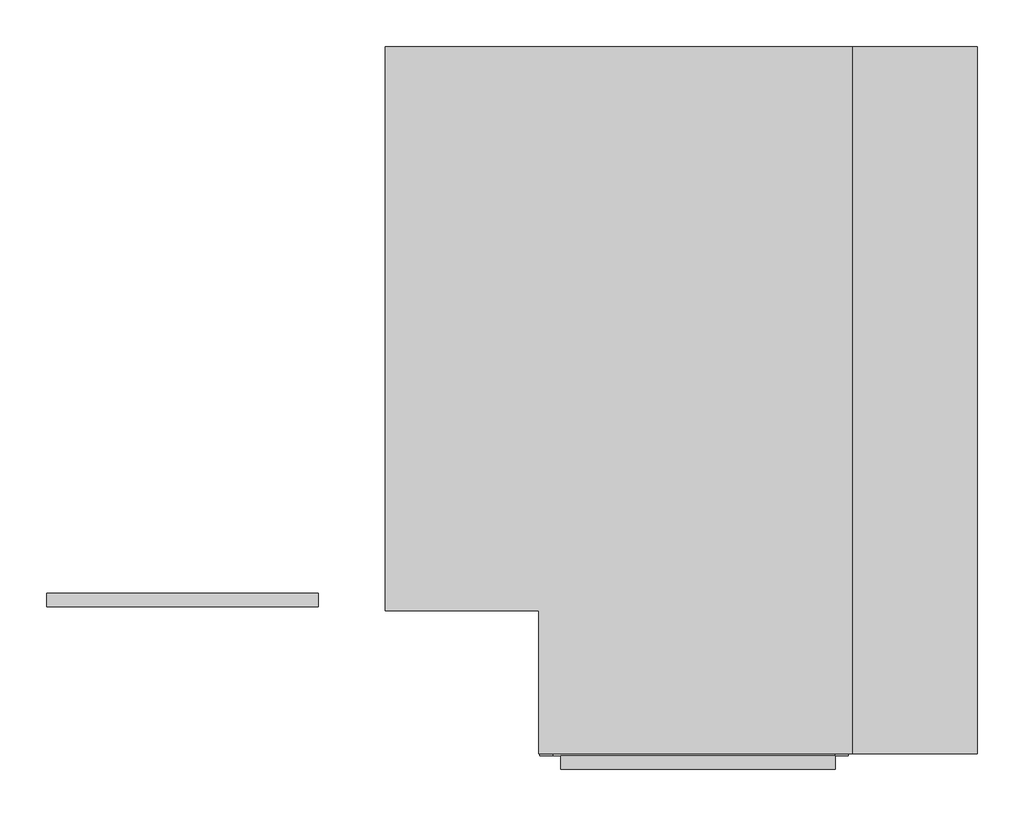
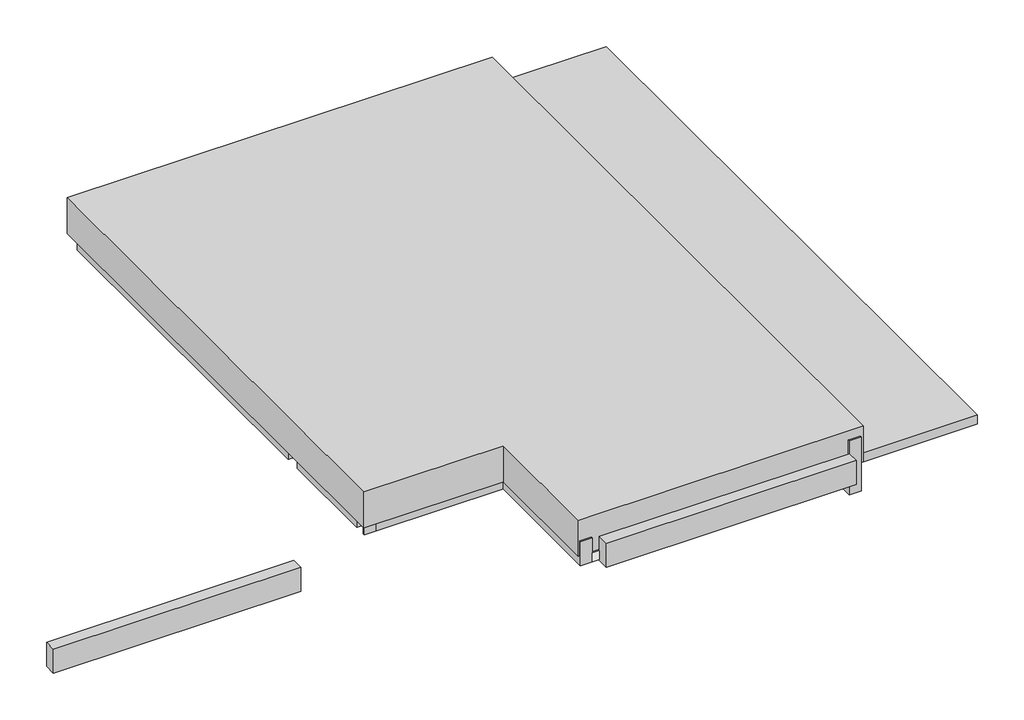
# One storey: 7 beams, 2 proxies, 2 slabs.
"""IFC4 building model written with IfcOpenShell, lengths in millimetres."""

from ifc_helpers import new_model, si_unit, frame, origin, place, context, project, spatial, polyline, circle_curve, ellipse_curve, outline, extrude, faceted_brep, element, save
from ifc_brep_helpers import plane_surface, cylinder_surface, revolved_surface, advanced_brep

model = new_model("IFC4")

# Units and contexts
model_context = context("Model", 3, world=origin())
ifc_project = project(units=[si_unit("LENGTHUNIT", "METRE", prefix="MILLI")], contexts=[model_context])

# Site, building, storey
site = spatial("IfcSite", under=ifc_project)
building = spatial("IfcBuilding", under=site)
storey = spatial("IfcBuildingStorey", under=building, Name="COBERTURA SALA DE ESTAR", Elevation=4400.0)

# Beams
placement = place(None, origin())
element("IfcBeam", 1, ObjectType="TQS - Viga retangular : 19.0 x 40.0", at=placement, inside=storey, context=model_context, shape_type="SweptSolid", body=[
    extrude(outline(polyline([(-7621.281307, -2044.5699847), (-7621.281307, -2234.5699847), (-11521.281307, -2234.5699847), (-11521.281307, -2044.5699847), (-7621.281307, -2044.5699847)])), frame((0.0, 0.0, 3640.0), z_axis=(0.0, 0.0, 1.0), x_axis=(1.0, 0.0, 0.0)), (0.0, 0.0, 1.0), 400.0),
])
element("IfcBeam", 2, ObjectType="TQS - Viga retangular : 19.0 x 40.0", at=placement, inside=storey, context=model_context, shape_type="SweptSolid", body=[
    extrude(outline(polyline([(-202.281307, -4375.5699847), (-202.281307, -4565.5699847), (-4142.481307, -4565.5699847), (-4142.481307, -4375.5699847), (-202.281307, -4375.5699847)])), frame((0.0, 0.0, 4240.0), z_axis=(0.0, 0.0, 1.0), x_axis=(1.0, 0.0, 0.0)), (0.0, 0.0, 1.0), 400.0),
])
element("IfcBeam", 3, ObjectType="TQS - Viga retangular : 19.0 x 40.0", at=placement, inside=storey, context=model_context, shape_type="Brep", body=[
    faceted_brep([(-4442.481307, -2259.5699847, 4650.0), (-4252.481307, -2259.5699847, 4650.0), (-4252.481307, -2259.5699847, 4400.0), (-4252.481307, -2259.5699847, 4250.0), (-4442.481307, -2259.5699847, 4250.0), (-4442.481307, -4375.5699847, 4650.0), (-4252.481307, -4375.5699847, 4650.0), (-4252.481307, -4375.5699847, 4400.0), (-4252.481307, -4375.5699847, 4250.0), (-4442.481307, -4375.5699847, 4250.0)], [[[0, 1, 2, 3, 4]], [[1, 0, 5, 6]], [[3, 2, 1, 6, 7, 8]], [[4, 3, 8, 9]], [[0, 4, 9, 5]], [[5, 9, 8, 7, 6]]]),
])
element("IfcBeam", 4, ObjectType="TQS - Viga retangular : 19.0 x 60.0", at=placement, inside=storey, context=model_context, shape_type="AdvancedBrep", body=[
    advanced_brep(
    [(-412.281307, 5774.4300153, 4850.0), (-6230.281307, 5774.4300153, 4850.0), (-6230.281307, 5620.2264681, 4850.0), (-6139.9212645, 5625.5330018, 4850.0), (-6117.841019, 5621.0415768, 4850.0), (-6230.281307, 5613.9936641, 4850.0), (-6230.281307, 5584.4300153, 4850.0), (-412.281307, 5584.4300153, 4850.0), (-412.281307, 5610.6528241, 4850.0), (-563.721595, 5621.0415768, 4850.0), (-541.6413494, 5625.5330018, 4850.0), (-412.281307, 5617.2895263, 4850.0), (-6230.281307, 5584.4300153, 4250.0), (-412.281307, 5584.4300153, 4250.0), (-6230.281307, 5774.4300153, 4250.0), (-412.281307, 5774.4300153, 4250.0), (-6230.281307, 5621.0415768, 4838.7559712), (-6230.281307, 5625.5330018, 4840.9639958), (-412.281307, 5625.5330018, 4837.0639958), (-412.281307, 5621.0415768, 4834.8559712)],
    [
        (0, 1),
        (1, 2),
        (2, 3, ellipse_curve(frame((-5844.9559183, 5565.5330018, 4850.0), z_axis=(0.0, 0.0, -1.0), x_axis=(-0.9999999999999999, 0.0, 0.0)), 671.270851, 66.7939461)),
        (3, 4),
        (4, 5, ellipse_curve(frame((-5844.9559183, 5565.5330018, 4850.0), z_axis=(0.0, 0.0, 1.0), x_axis=(-0.9999999999999999, 0.0, 0.0)), 621.0214729, 61.7939461)),
        (5, 6),
        (6, 7),
        (7, 8),
        (8, 9, ellipse_curve(frame((-836.6066956, 5565.5330018, 4850.0), z_axis=(0.0, 0.0, 1.0), x_axis=(-0.9999999999999999, 0.0, 0.0)), 621.0214729, 61.7939461)),
        (9, 10),
        (10, 11, ellipse_curve(frame((-836.6066956, 5565.5330018, 4850.0), z_axis=(0.0, 0.0, -1.0), x_axis=(-0.9999999999999999, 0.0, 0.0)), 671.270851, 66.7939461)),
        (11, 0),
        (6, 12),
        (12, 13),
        (13, 7),
        (12, 14),
        (14, 15),
        (15, 13),
        (0, 15),
        (14, 1),
        (5, 16, ellipse_curve(frame((-6230.281307, 5565.5330018, 4811.4674611), z_axis=(-1.0, 0.0, 0.0), x_axis=(0.0, 0.0, -1.0)), 62.1021473, 61.7939461)),
        (16, 17),
        (17, 2, ellipse_curve(frame((-6230.281307, 5565.5330018, 4811.4674611), z_axis=(1.0, 0.0, 0.0), x_axis=(0.0, 0.0, -1.0)), 67.1270851, 66.7939461)),
        (11, 18, ellipse_curve(frame((-412.281307, 5565.5330018, 4807.5674611), z_axis=(-1.0, 0.0, 0.0), x_axis=(0.0, 0.0, 1.0)), 67.1270851, 66.7939461)),
        (18, 19),
        (19, 8, ellipse_curve(frame((-412.281307, 5565.5330018, 4807.5674611), z_axis=(1.0, 0.0, 0.0), x_axis=(0.0, 0.0, 1.0)), 62.1021473, 61.7939461)),
        (4, 16),
        (3, 17),
        (19, 9),
        (18, 10),
    ],
    [
        plane_surface(frame((-424.9813076, 5774.4300153, 4850.0), z_axis=(0.0, 0.0, 1.0), x_axis=(-1.0, 0.0, 0.0))),
        plane_surface(frame((-424.9813076, 5584.4300153, 4850.0), z_axis=(0.0, -1.0, 0.0), x_axis=(-1.0, 0.0, 0.0))),
        plane_surface(frame((-424.9813076, 5584.4300153, 4250.0), z_axis=(0.0, 0.0, -1.0), x_axis=(-1.0, 0.0, 0.0))),
        plane_surface(frame((-424.9813076, 5774.4300153, 4250.0), z_axis=(0.0, 1.0, 0.0), x_axis=(-1.0, 0.0, 0.0))),
        plane_surface(frame((-6230.281307, 5679.4300153, 4850.0), z_axis=(-1.0, 0.0, 0.0), x_axis=(0.0, -1.0, 0.0))),
        plane_surface(frame((-412.281307, 5679.4300153, 4850.0), z_axis=(1.0, 0.0, 0.0), x_axis=(0.0, 1.0, 0.0))),
        cylinder_surface(frame((-3344.074248, 5565.5330018, 5100.088167), z_axis=(-0.9950371902099892, 0.0, -0.09950371902099951), x_axis=(-0.0893826983688466, 0.4394133093826145, 0.8938269836885228)), 61.7939461),
        plane_surface(frame((-3346.8853889, 5623.2872893, 5128.1995753), z_axis=(-0.08938269836887112, -0.4394133093823482, 0.8938269836886512), x_axis=(-0.043723258470857625, 0.8982850012872601, 0.4372325847086854))),
        revolved_surface(polyline([(-6515.550746384648, 5536.182852897475, 4843.239770846461), (-5186.301536483657, 5536.182852897475, 4976.164691836561)]), (-3344.074248, 5565.5330018, 5100.088167), (-0.9950371902099892, 0.0, -0.09950371902099951)),
        cylinder_surface(frame((-379.7327874, 5565.5330018, 4804.3126092), z_axis=(-0.9950371902099892, 0.0, 0.09950371902099964), x_axis=(0.08938269836885342, 0.43941330938261464, 0.893826983688522)), 61.7939461),
        plane_surface(frame((-376.9216465, 5623.2872893, 4832.4240174), z_axis=(0.08938269836886582, -0.43941330938234807, 0.8938269836886518), x_axis=(0.04372325847086866, 0.8982850012872601, 0.4372325847086842))),
        revolved_surface(polyline([(-1495.2610774113932, 5536.182852897475, 4976.164691886069), (-166.01186751040316, 5536.182852897475, 4843.239770895969)]), (-379.7327874, 5565.5330018, 4804.3126092), (-0.9950371902099892, 0.0, 0.09950371902099964)),
    ],
    [
        (0, [[1, 2, 3, 4, 5, 6, 7, 8, 9, 10, 11, 12]]),
        (1, [[-7, 13, 14, 15]]),
        (2, [[-14, 16, 17, 18]]),
        (3, [[-1, 19, -17, 20]]),
        (4, [[-20, -16, -13, -6, 21, 22, 23, -2]]),
        (5, [[-15, -18, -19, -12, 24, 25, 26, -8]]),
        (6, [[27, -21, -5]]),
        (7, [[-27, -4, 28, -22]]),
        (8, [[-28, -3, -23]]),
        (9, [[29, -9, -26]]),
        (10, [[-29, -25, 30, -10]]),
        (11, [[-30, -24, -11]]),
    ],
),
])
element("IfcBeam", 5, ObjectType="TQS - Viga retangular : 19.0 x 60.0", at=placement, inside=storey, context=model_context, shape_type="Brep", body=[
    faceted_brep([(-6630.281307, -174.5699847, 4850.0), (-6440.281307, -174.5699847, 4850.0), (-6440.281307, 5584.4300153, 4850.0), (-6630.281307, 5584.4300153, 4850.0), (-6440.281307, -174.5699847, 4250.0), (-6440.281307, 5584.4300153, 4250.0), (-6440.281307, 5584.4300153, 4400.0), (-6630.281307, -174.5699847, 4250.0), (-6630.281307, 5584.4300153, 4250.0)], [[[0, 1, 2, 3]], [[1, 4, 5, 6, 2]], [[4, 7, 8, 5]], [[7, 0, 3, 8]], [[1, 0, 7, 4]], [[3, 2, 6, 5, 8]]]),
    faceted_brep([(-6630.281307, -424.5699847, 4850.0), (-6440.281307, -424.5699847, 4850.0), (-6440.281307, -424.5699847, 4250.0), (-6630.281307, -424.5699847, 4250.0), (-6630.281307, -2044.5699847, 4850.0), (-6440.281307, -2044.5699847, 4850.0), (-6440.281307, -2044.5699847, 4250.0), (-6630.281307, -2044.5699847, 4250.0)], [[[0, 1, 2, 3]], [[1, 0, 4, 5]], [[2, 1, 5, 6]], [[3, 2, 6, 7]], [[0, 3, 7, 4]], [[5, 4, 7, 6]]]),
    faceted_brep([(-6440.281307, -2259.5699847, 4850.0), (-6630.281307, -2259.5699847, 4850.0), (-6630.281307, -2259.5699847, 4250.0), (-6440.281307, -2259.5699847, 4250.0), (-6630.281307, -2234.5699847, 4850.0), (-6440.281307, -2234.5699847, 4850.0), (-6440.281307, -2234.5699847, 4250.0), (-6630.281307, -2234.5699847, 4250.0)], [[[0, 1, 2, 3]], [[4, 5, 6, 7]], [[1, 0, 5, 4]], [[0, 3, 6, 5]], [[3, 2, 7, 6]], [[2, 1, 4, 7]]]),
])
element("IfcBeam", 6, ObjectType="TQS - Viga retangular : 19.0 x 60.0", at=placement, inside=storey, context=model_context, shape_type="AdvancedBrep", body=[
    advanced_brep(
    [(-202.6220088, -2259.5699847, 4850.0), (-202.6137562, -2069.5699847, 4850.0), (-6440.281307, -2069.5699847, 4850.0), (-6440.281307, -2234.5699847, 4850.0), (-6440.281307, -2259.5699847, 4850.0), (-375.1640483, -2209.9569973, 4850.0), (-375.1640483, -2217.1114577, 4850.0), (-563.721595, -2202.9584232, 4850.0), (-541.6413494, -2198.4669982, 4850.0), (-202.6220088, -2259.5699847, 4250.0), (-202.6220088, -2259.5699847, 4400.0), (-6440.281307, -2259.5699847, 4250.0), (-4442.481307, -2259.5699847, 4250.0), (-4252.481307, -2259.5699847, 4250.0), (-202.6137562, -2069.5699847, 4250.0), (-6440.281307, -2234.5699847, 4250.0), (-6440.281307, -2069.5699847, 4250.0), (-202.6137562, -2069.5699847, 4400.0), (-6440.281307, -2069.5699847, 4400.0), (-376.8123384, -2198.4669982, 4833.5170989), (-377.0309547, -2202.9584232, 4831.330936)],
    [
        (0, 1),
        (1, 2),
        (2, 3),
        (3, 4),
        (4, 0),
        (5, 6),
        (6, 7, ellipse_curve(frame((-836.6066956, -2258.4669982, 4850.0), z_axis=(0.0, 0.0, 1.0), x_axis=(-0.9999999999999999, 0.0, 0.0)), 621.0214729, 61.7939461)),
        (7, 8),
        (8, 5, ellipse_curve(frame((-836.6066956, -2258.4669982, 4850.0), z_axis=(0.0, 0.0, -1.0), x_axis=(-0.9999999999999999, 0.0, 0.0)), 671.270851, 66.7939461)),
        (9, 10),
        (10, 0),
        (4, 11),
        (11, 12),
        (12, 13),
        (13, 9),
        (14, 9),
        (11, 15),
        (15, 16),
        (16, 14),
        (1, 17),
        (17, 14),
        (16, 18),
        (18, 2),
        (19, 20),
        (20, 6, circle_curve(frame((-379.7327874, -2258.4669982, 4804.3126092), z_axis=(0.9950371902099892, 0.0, -0.09950371902099961), x_axis=(0.08938269836885339, 0.4394133093826145, 0.893826983688522)), 61.7939461)),
        (5, 19, circle_curve(frame((-379.7327874, -2258.4669982, 4804.3126092), z_axis=(-0.9950371902099892, 0.0, 0.09950371902099961), x_axis=(0.08938269836885117, -0.4394133093826303, 0.8938269836885144)), 66.7939461)),
        (20, 7),
        (19, 8),
    ],
    [
        plane_surface(frame((-215.3220088, -2069.5699847, 4850.0), z_axis=(0.0, 0.0, 1.0), x_axis=(-1.0, 0.0, 0.0))),
        plane_surface(frame((-215.3220088, -2259.5699847, 4850.0), z_axis=(0.0, -1.0, 0.0), x_axis=(-1.0, 0.0, 0.0))),
        plane_surface(frame((-215.3220088, -2259.5699847, 4250.0), z_axis=(0.0, 0.0, -1.0), x_axis=(-1.0, 0.0, 0.0))),
        plane_surface(frame((-215.3220088, -2069.5699847, 4250.0), z_axis=(0.0, 1.0, 0.0), x_axis=(-1.0, 0.0, 0.0))),
        plane_surface(frame((-6440.281307, -2234.5699847, 4850.0), z_axis=(-1.0, 0.0, 0.0), x_axis=(0.0, 0.0, -1.0))),
        plane_surface(frame((-202.2818588, 5571.7300153, 3950.0), z_axis=(0.9999999990567141, -4.343468567533895e-05, 0.0), x_axis=(-4.343468567533895e-05, -0.9999999990567141, 0.0))),
        plane_surface(frame((-373.8918894, -2311.673052, 4862.7215886), z_axis=(-0.9950371902099892, 0.0, 0.09950371902099943), x_axis=(-0.09950371902099943, 0.0, -0.9950371902099892))),
        cylinder_surface(frame((-379.7327874, -2258.4669982, 4804.3126092), z_axis=(-0.9950371902099892, 0.0, 0.09950371902099961), x_axis=(0.08938269836885339, 0.4394133093826145, 0.893826983688522)), 61.7939461),
        plane_surface(frame((-376.9216465, -2200.7127107, 4832.4240174), z_axis=(0.0893826983688658, -0.4394133093823482, 0.8938269836886518), x_axis=(0.04372325847086866, 0.8982850012872601, 0.4372325847086843))),
        revolved_surface(polyline([(-1495.2610774113932, -2287.817147102526, 4976.164691886069), (-166.01186751040316, -2287.817147102526, 4843.239770895969)]), (-379.7327874, -2258.4669982, 4804.3126092), (-0.9950371902099892, 0.0, 0.09950371902099961)),
    ],
    [
        (0, [[1, 2, 3, 4, 5], [6, 7, 8, 9]]),
        (1, [[10, 11, -5, 12, 13, 14, 15]]),
        (2, [[16, -15, -14, -13, 17, 18, 19]]),
        (3, [[20, 21, -19, 22, 23, -2]]),
        (4, [[-23, -22, -18, -17, -12, -4, -3]]),
        (5, [[-1, -11, -10, -16, -21, -20]]),
        (6, [[24, 25, -6, 26]]),
        (7, [[-25, 27, -7]]),
        (8, [[-24, 28, -8, -27]]),
        (9, [[-26, -9, -28]]),
    ],
),
])
element("IfcBeam", 7, ObjectType="TQS - Viga retangular : 19.0 x 90.0", at=placement, inside=storey, context=model_context, shape_type="Brep", body=[
    faceted_brep([(-12.281307, 5584.4300153, 4850.0), (-202.2813068, 5584.4382679, 4850.0), (-202.6137562, -2069.5699847, 4850.0), (-202.6220088, -2259.5699847, 4850.0), (-202.7139163, -4375.561732, 4850.0), (-12.7139164, -4375.5699846, 4850.0), (-12.281307, 5584.4300153, 3950.0), (-12.7139164, -4375.5699846, 3950.0), (-202.2813068, 5584.4382679, 3950.0), (-202.7139163, -4375.561732, 3950.0)], [[[0, 1, 2, 3, 4, 5]], [[6, 0, 5, 7]], [[8, 6, 7, 9]], [[1, 8, 9, 4, 3, 2]], [[1, 0, 6, 8]], [[4, 9, 7, 5]]]),
])

# Proxies
element("IfcBuildingElementProxy", 8, Name="PERGOLADO SALAS1 : PERGOLADO SALAS", ObjectType="PERGOLADO SALAS1 : PERGOLADO SALAS", at=placement, inside=storey, context=model_context, shape_type="SweptSolid", body=[
    extrude(outline(polyline([(1839.718693, 5804.4300153), (1839.718693, -4345.5699847), (39.718693, -4345.5699847), (39.718693, 5804.4300153), (1839.718693, 5804.4300153)])), frame((0.0, 0.0, 4400.0), z_axis=(0.0, 0.0, 1.0), x_axis=(1.0, 0.0, 0.0)), (0.0, 0.0, 1.0), 150.0),
])
element("IfcBuildingElementProxy", 9, Name="COBERTURA SALA DE ESTAR : COBERTURA SALA DE ESTAR", ObjectType="COBERTURA SALA DE ESTAR : COBERTURA SALA DE ESTAR", at=placement, inside=storey, context=model_context, shape_type="SweptSolid", body=[
    extrude(outline(polyline([(39.718693, 5804.4300153), (39.718693, -4345.5699847), (-4457.4976512, -4345.5699847), (-4457.4976512, -2295.5699847), (-6660.281307, -2295.5699847), (-6660.281307, 5804.4300153), (39.718693, 5804.4300153)])), frame((0.0, 0.0, 4400.0), z_axis=(0.0, 0.0, 1.0), x_axis=(1.0, 0.0, 0.0)), (0.0, 0.0, 1.0), 600.0),
])

# Slabs
element("IfcSlab", 10, ObjectType="TQS h=15", at=placement, inside=storey, context=model_context, shape_type="Brep", body=[
    faceted_brep([(-6440.281307, -2069.5699847, 4250.0), (-6440.281307, -2044.5699847, 4250.0), (-6440.281307, -424.5699847, 4250.0), (-6440.281307, -174.5699847, 4250.0), (-6440.281307, 5584.4300153, 4250.0), (-6230.281307, 5584.4300153, 4250.0), (-412.281307, 5584.4300153, 4250.0), (-202.2813071, 5584.4300153, 4250.0), (-202.6137562, -2069.5699847, 4250.0), (-6440.281307, -2069.5699847, 4400.0), (-202.6137562, -2069.5699847, 4400.0), (-202.2813071, 5584.4300153, 4400.0), (-6440.281307, 5584.4300153, 4400.0)], [[[0, 1, 2, 3, 4, 5, 6, 7, 8]], [[9, 10, 11, 12]], [[4, 3, 2, 1, 0, 9, 12]], [[7, 6, 5, 4, 12, 11]], [[8, 7, 11, 10]], [[0, 8, 10, 9]]]),
])
element("IfcSlab", 11, ObjectType="TQS h=15", at=placement, inside=storey, context=model_context, shape_type="SweptSolid", body=[
    extrude(outline(polyline([(-202.6220088, -2259.5699847), (-202.7139166, -4375.5699847), (-4252.481307, -4375.5699847), (-4252.481307, -2259.5699847), (-202.6220088, -2259.5699847)])), frame((0.0, 0.0, 4250.0), z_axis=(0.0, 0.0, 1.0), x_axis=(1.0, 0.0, 0.0)), (0.0, 0.0, 1.0), 150.0),
])

save(model, "model.ifc")

# Revit data of these elements
# Type "TQS - Viga retangular : 19.0 x 40.0"
#   Length [instance default] = 1.524 m
#   b = 0.19 m
#   h = 0.40 m
#   Structural Material [instance default] = none
#   Assembly Code = ""
# Type "TQS - Viga retangular : 19.0 x 60.0"
#   Length [instance default] = 1.524 m
#   b = 0.19 m
#   h = 0.60 m
#   Structural Material [instance default] = none
#   Assembly Code = ""
# Type "TQS - Viga retangular : 19.0 x 90.0"
#   Length [instance default] = 1.524 m
#   b = 0.19 m
#   h = 0.90 m
#   Structural Material [instance default] = none
#   Assembly Code = ""
# Type "TQS h=15"
#   Function = 0
#   Layers, outside or top first: 0.15 m ".MATERIAL GENÉRICO LAJE E PISO" (function 1)
# Element 1 (IfcBeam, "TQS - Viga retangular : 19.0 x 40.0")
#   Uso = "ESTRUTURA"
#   Titulo = "V302"
#   Chave = "-194"
#   Tipo Elemento = "Viga"
#   SHA1 = "623FD7AF7D5DA8F9D9CA08F45AA7E3989112ED0B"
#   Revisão = ""
#   Tipo de carga = ""
#   Divisor de flexao = ""
#   Secao = ""
#   Configuracao = ""
#   Angulo (graus) = ""
#   Detalhamento = ""
#   Casos de vento manual = ""
#   Tipo = ""
#   Alcas = ""
#   Furos = ""
#   Pino = ""
#   Distribuicao = ""
#   Solidarizado = ""
#   Solidarizar na montagem = ""
#   Unir com o próximo = ""
#   Grupo pre moldado = ""
#   Verificado = ""
#   Concreto C = ""
#   Taxa de armadura (kgf/m³) = 0
#   Carga (tf/m²) = 0
#   Carga (tf/m) = 0
#   Carga (tf) = 0
#   Altura = 0.40 m
#   Rebaixo = 0.36 m
#   Largura = 0.19 m
#   Distancia a face = 0.00 m
#   Distancia ao eixo = 0.00 m
#   Altura gerber esquerda = 0.00 m
#   Largura gerber esquerda = 0.00 m
#   Altura gerber direita = 0.00 m
#   Largura gerber direita = 0.00 m
#   Resultado de Ensaios fck (MPa) = 0
#   Unique TQS ID = -194
#   Principal = yes
#   Structural Material = none
#   Phase Created = CC_AP/ESTR
# Element 2 (IfcBeam, "TQS - Viga retangular : 19.0 x 40.0")
#   Uso = "ESTRUTURA"
#   Titulo = "V304"
#   Chave = "-347"
#   Tipo Elemento = "Viga"
#   SHA1 = "DE726C8B00042777CE20FAEC480409A8753BC175"
#   Revisão = ""
#   Tipo de carga = ""
#   Divisor de flexao = ""
#   Secao = ""
#   Configuracao = ""
#   Angulo (graus) = ""
#   Detalhamento = ""
#   Casos de vento manual = ""
#   Tipo = ""
#   Alcas = ""
#   Furos = ""
#   Pino = ""
#   Distribuicao = ""
#   Solidarizado = ""
#   Solidarizar na montagem = ""
#   Unir com o próximo = ""
#   Grupo pre moldado = ""
#   Verificado = ""
#   Concreto C = ""
#   Taxa de armadura (kgf/m³) = 0
#   Carga (tf/m²) = 0
#   Carga (tf/m) = 0
#   Carga (tf) = 0
#   Altura = 0.40 m
#   Rebaixo = -0.24 m
#   Largura = 0.19 m
#   Distancia a face = 0.00 m
#   Distancia ao eixo = 0.00 m
#   Altura gerber esquerda = 0.00 m
#   Largura gerber esquerda = 0.00 m
#   Altura gerber direita = 0.00 m
#   Largura gerber direita = 0.00 m
#   Resultado de Ensaios fck (MPa) = 0
#   Unique TQS ID = -347
#   Principal = yes
#   Structural Material = none
#   Phase Created = CC_AP/ESTR
# Element 3 (IfcBeam, "TQS - Viga retangular : 19.0 x 40.0")
#   Uso = "ESTRUTURA"
#   Titulo = "V306"
#   Chave = "-348"
#   Tipo Elemento = "Viga"
#   SHA1 = "0486A55721C7CA422F82DF13CBABE904850BDE6D"
#   Revisão = ""
#   Tipo de carga = ""
#   Divisor de flexao = ""
#   Secao = ""
#   Configuracao = ""
#   Angulo (graus) = ""
#   Detalhamento = ""
#   Casos de vento manual = ""
#   Tipo = ""
#   Alcas = ""
#   Furos = ""
#   Pino = ""
#   Distribuicao = ""
#   Solidarizado = ""
#   Solidarizar na montagem = ""
#   Unir com o próximo = ""
#   Grupo pre moldado = ""
#   Verificado = ""
#   Concreto C = ""
#   Taxa de armadura (kgf/m³) = 0
#   Carga (tf/m²) = 0
#   Carga (tf/m) = 0
#   Carga (tf) = 0
#   Altura = 0.40 m
#   Rebaixo = -0.25 m
#   Largura = 0.19 m
#   Distancia a face = 0.00 m
#   Distancia ao eixo = 0.00 m
#   Altura gerber esquerda = 0.00 m
#   Largura gerber esquerda = 0.00 m
#   Altura gerber direita = 0.00 m
#   Largura gerber direita = 0.00 m
#   Resultado de Ensaios fck (MPa) = 0
#   Unique TQS ID = -348
#   Principal = yes
#   Structural Material = none
#   Phase Created = CC_AP/ESTR
# Element 4 (IfcBeam, "TQS - Viga retangular : 19.0 x 60.0")
#   Uso = "ESTRUTURA"
#   Titulo = "V301"
#   Chave = "-296"
#   Tipo Elemento = "Viga"
#   SHA1 = "757894CEA72A4CB6221DF2E576041B09F085C368"
#   Revisão = ""
#   Tipo de carga = ""
#   Divisor de flexao = ""
#   Secao = ""
#   Configuracao = ""
#   Angulo (graus) = ""
#   Detalhamento = ""
#   Casos de vento manual = ""
#   Tipo = ""
#   Alcas = ""
#   Furos = ""
#   Pino = ""
#   Distribuicao = ""
#   Solidarizado = ""
#   Solidarizar na montagem = ""
#   Unir com o próximo = ""
#   Grupo pre moldado = ""
#   Verificado = ""
#   Concreto C = ""
#   Taxa de armadura (kgf/m³) = 0
#   Carga (tf/m²) = 0
#   Carga (tf/m) = 0
#   Carga (tf) = 0
#   Altura = 0.60 m
#   Rebaixo = -0.45 m
#   Largura = 0.19 m
#   Distancia a face = 0.00 m
#   Distancia ao eixo = 0.00 m
#   Altura gerber esquerda = 0.00 m
#   Largura gerber esquerda = 0.00 m
#   Altura gerber direita = 0.00 m
#   Largura gerber direita = 0.00 m
#   Resultado de Ensaios fck (MPa) = 0
#   Unique TQS ID = -296
#   Principal = yes
#   Structural Material = none
#   Phase Created = CC_AP/ESTR
# Element 5 (IfcBeam, "TQS - Viga retangular : 19.0 x 60.0")
#   Uso = "ESTRUTURA"
#   Titulo = "V305"
#   Chave = "-297"
#   Tipo Elemento = "Viga"
#   SHA1 = "BDE1024E341324ECB798242B9C26029271E807E6"
#   Revisão = ""
#   Tipo de carga = ""
#   Divisor de flexao = ""
#   Secao = ""
#   Configuracao = ""
#   Angulo (graus) = ""
#   Detalhamento = ""
#   Casos de vento manual = ""
#   Tipo = ""
#   Alcas = ""
#   Furos = ""
#   Pino = ""
#   Distribuicao = ""
#   Solidarizado = ""
#   Solidarizar na montagem = ""
#   Unir com o próximo = ""
#   Grupo pre moldado = ""
#   Verificado = ""
#   Concreto C = ""
#   Taxa de armadura (kgf/m³) = 0
#   Carga (tf/m²) = 0
#   Carga (tf/m) = 0
#   Carga (tf) = 0
#   Altura = 0.60 m
#   Rebaixo = -0.45 m
#   Largura = 0.19 m
#   Distancia a face = 0.00 m
#   Distancia ao eixo = 0.00 m
#   Altura gerber esquerda = 0.00 m
#   Largura gerber esquerda = 0.00 m
#   Altura gerber direita = 0.00 m
#   Largura gerber direita = 0.00 m
#   Resultado de Ensaios fck (MPa) = 0
#   Unique TQS ID = -297
#   Principal = yes
#   Structural Material = none
#   Phase Created = CC_AP/ESTR
# Element 6 (IfcBeam, "TQS - Viga retangular : 19.0 x 60.0")
#   Uso = "ESTRUTURA"
#   Titulo = "V303"
#   Chave = "-345"
#   Tipo Elemento = "Viga"
#   SHA1 = "033B8EC3397B601DC3ABF9BA590BF3ACBC45E410"
#   Revisão = ""
#   Tipo de carga = ""
#   Divisor de flexao = ""
#   Secao = ""
#   Configuracao = ""
#   Angulo (graus) = ""
#   Detalhamento = ""
#   Casos de vento manual = ""
#   Tipo = ""
#   Alcas = ""
#   Furos = ""
#   Pino = ""
#   Distribuicao = ""
#   Solidarizado = ""
#   Solidarizar na montagem = ""
#   Unir com o próximo = ""
#   Grupo pre moldado = ""
#   Verificado = ""
#   Concreto C = ""
#   Taxa de armadura (kgf/m³) = 0
#   Carga (tf/m²) = 0
#   Carga (tf/m) = 0
#   Carga (tf) = 0
#   Altura = 0.60 m
#   Rebaixo = -0.45 m
#   Largura = 0.19 m
#   Distancia a face = 0.00 m
#   Distancia ao eixo = 0.00 m
#   Altura gerber esquerda = 0.00 m
#   Largura gerber esquerda = 0.00 m
#   Altura gerber direita = 0.00 m
#   Largura gerber direita = 0.00 m
#   Resultado de Ensaios fck (MPa) = 0
#   Unique TQS ID = -345
#   Principal = yes
#   Structural Material = none
#   Phase Created = CC_AP/ESTR
# Element 7 (IfcBeam, "TQS - Viga retangular : 19.0 x 90.0")
#   Uso = "ESTRUTURA"
#   Titulo = "V307"
#   Chave = "-298"
#   Tipo Elemento = "Viga"
#   SHA1 = "4A4DC69E98A9D766DC72AD6B038202D9AEA1F49E"
#   Revisão = ""
#   Tipo de carga = ""
#   Divisor de flexao = ""
#   Secao = ""
#   Configuracao = ""
#   Angulo (graus) = ""
#   Detalhamento = ""
#   Casos de vento manual = ""
#   Tipo = ""
#   Alcas = ""
#   Furos = ""
#   Pino = ""
#   Distribuicao = ""
#   Solidarizado = ""
#   Solidarizar na montagem = ""
#   Unir com o próximo = ""
#   Grupo pre moldado = ""
#   Verificado = ""
#   Concreto C = ""
#   Taxa de armadura (kgf/m³) = 0
#   Carga (tf/m²) = 0
#   Carga (tf/m) = 0
#   Carga (tf) = 0
#   Altura = 0.90 m
#   Rebaixo = -0.45 m
#   Largura = 0.19 m
#   Distancia a face = 0.00 m
#   Distancia ao eixo = 0.00 m
#   Altura gerber esquerda = 0.00 m
#   Largura gerber esquerda = 0.00 m
#   Altura gerber direita = 0.00 m
#   Largura gerber direita = 0.00 m
#   Resultado de Ensaios fck (MPa) = 0
#   Unique TQS ID = -298
#   Principal = yes
#   Structural Material = none
#   Phase Created = CC_AP/ESTR
# Element 8 (IfcBuildingElementProxy, "PERGOLADO SALAS1 : PERGOLADO SALAS")
#   Phase Created = CC_COMPLETO
#   Materials on its faces: "Forma padrão"
# Element 9 (IfcBuildingElementProxy, "COBERTURA SALA DE ESTAR : COBERTURA SALA DE ESTAR")
#   Phase Created = CC_EV
#   Materials on its faces: "Forma padrão"
# Element 10 (IfcSlab, "TQS h=15")
#   Uso = "ESTRUTURA"
#   Titulo = "L1"
#   Chave = "-343"
#   Tipo Elemento = "Laje"
#   SHA1 = "CBCB75B0B1E6306AA97FD72F3CCB2019DA0CDC21"
#   Revisão = ""
#   Tipo de carga = ""
#   Divisor de flexao = ""
#   Fabricante = ""
#   Enchimento = ""
#   Mini painel = ""
#   Blocos por nervura = ""
#   Secao = ""
#   Configuracao = ""
#   Angulo (graus) = "0"
#   Detalhamento = ""
#   Casos de vento manual = ""
#   Tipo = "Pré-moldada"
#   Alcas = ""
#   Furos = ""
#   Pino = ""
#   Distribuicao = ""
#   Solidarizado = ""
#   Solidarizar na montagem = ""
#   Unir com o próximo = ""
#   Grupo pre moldado = ""
#   Verificado = ""
#   Concreto C = ""
#   Height Offset From Level = 0.00 m
#   Taxa de armadura (kgf/m³) = 0
#   Carga (tf/m²) = 0
#   Carga (tf/m) = 0
#   Carga (tf) = 0
#   Altura = 0.15 m
#   Capa = 0.04 m
#   Capa inferior = 0.00 m
#   Altura da nervura = 0.11 m
#   Enchimento (tf/m³) = 0.02
#   Largura inferior X = 0.00 m
#   Distancia inferior X = 0.00 m
#   Largura inferior Y = 0.00 m
#   Distancia inferior Y = 0.00 m
#   Largura vigota = 0.00 m
#   Altura vigota = 0.00 m
#   Largura perfil = 0.00 m
#   Largura aba = 0.00 m
#   Altura perfil = 0.00 m
#   Nervura secundaria = 0.00 m
#   Desconto nervura secundaria = 0.00 m
#   Rebaixo = 0.00 m
#   Largura = 0.00 m
#   Distancia a face = 0.00 m
#   Distancia ao eixo = 0.00 m
#   Resultado de Ensaios fck (MPa) = 0
#   built-in parameter 1001954 = 1
#   Unique TQS ID = -343
#   Principal = yes
#   Phase Created = CC_AP/ESTR
#   Materials on its faces: ".MATERIAL GENÉRICO LAJE E PISO"
# Element 11 (IfcSlab, "TQS h=15")
#   Uso = "ESTRUTURA"
#   Titulo = "L2"
#   Chave = "-344"
#   Tipo Elemento = "Laje"
#   SHA1 = "B69E32F9CB7C87F86F0BE6D4DE0B78773B0CC6FF"
#   Revisão = ""
#   Tipo de carga = ""
#   Divisor de flexao = ""
#   Fabricante = ""
#   Enchimento = ""
#   Mini painel = ""
#   Blocos por nervura = ""
#   Secao = ""
#   Configuracao = ""
#   Angulo (graus) = "90"
#   Detalhamento = ""
#   Casos de vento manual = ""
#   Tipo = "Pré-moldada"
#   Alcas = ""
#   Furos = ""
#   Pino = ""
#   Distribuicao = ""
#   Solidarizado = ""
#   Solidarizar na montagem = ""
#   Unir com o próximo = ""
#   Grupo pre moldado = ""
#   Verificado = ""
#   Concreto C = ""
#   Height Offset From Level = 0.00 m
#   Taxa de armadura (kgf/m³) = 0
#   Carga (tf/m²) = 0
#   Carga (tf/m) = 0
#   Carga (tf) = 0
#   Altura = 0.15 m
#   Capa = 0.04 m
#   Capa inferior = 0.00 m
#   Altura da nervura = 0.11 m
#   Enchimento (tf/m³) = 0.02
#   Largura inferior X = 0.00 m
#   Distancia inferior X = 0.00 m
#   Largura inferior Y = 0.00 m
#   Distancia inferior Y = 0.00 m
#   Largura vigota = 0.00 m
#   Altura vigota = 0.00 m
#   Largura perfil = 0.00 m
#   Largura aba = 0.00 m
#   Altura perfil = 0.00 m
#   Nervura secundaria = 0.00 m
#   Desconto nervura secundaria = 0.00 m
#   Rebaixo = 0.00 m
#   Largura = 0.00 m
#   Distancia a face = 0.00 m
#   Distancia ao eixo = 0.00 m
#   Resultado de Ensaios fck (MPa) = 0
#   built-in parameter 1001954 = 1
#   Unique TQS ID = -344
#   Principal = yes
#   Phase Created = CC_AP/ESTR
#   Materials on its faces: ".MATERIAL GENÉRICO LAJE E PISO"
# Materials
#   ".MATERIAL GENÉRICO LAJE E PISO": class ".CC_PAVIMENTAÇÃO", colour RGB 128 128 128, transparency 0, Description = "Material genérico para representação ND 200.", Cost = 0
#   "Forma padrão": class "Genérico", colour RGB 185 189 196, transparency 0.5, Cost = 0
